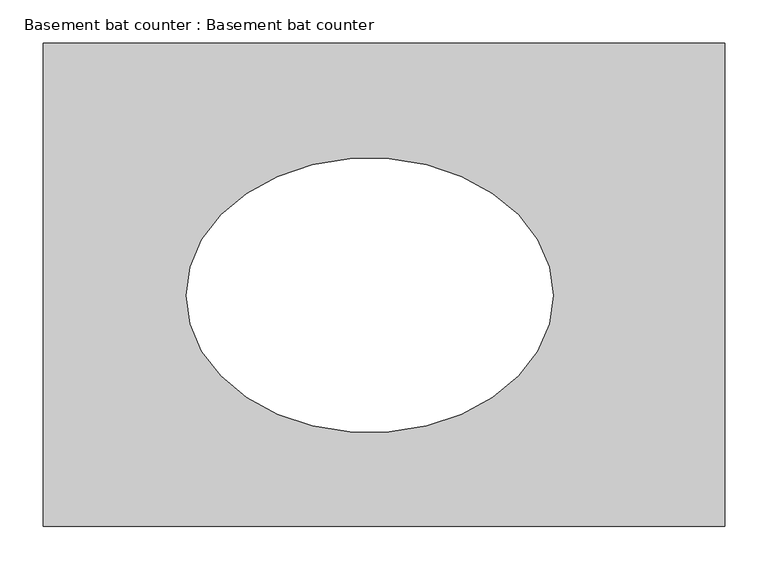
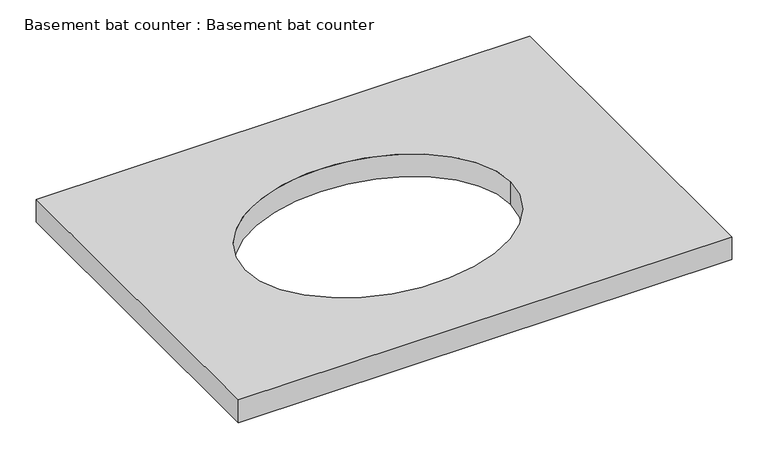
"""IFC4 building model written with IfcOpenShell, lengths in millimetres: furniture geometry, Basement bat counter : Basement bat counter."""

from ifc_helpers import new_model, si_unit, point, frame, origin, place, context, project, spatial, ellipse_curve, trimmed, source, transform, mapped, element, save
from ifc_brep_helpers import plane_surface, extruded_surface, advanced_brep


def basement_bat_counter_basement_bat_counter_ad1241f1(model_context):
    return source(origin(), model_context, "Body", "AdvancedBrep", [
        advanced_brep(
        [(963.0652851, 15145.821245, -2755.9), (963.0652851, 15704.621245, -2755.9), (1750.4652851, 15704.621245, -2755.9), (1750.4652851, 15145.821245, -2755.9), (1552.1234749, 15413.0467639, -2755.9), (1128.1234749, 15413.0467639, -2755.9), (963.0652851, 15145.821245, -2717.8), (1750.4652851, 15145.821245, -2717.8), (1750.4652851, 15704.621245, -2717.8), (963.0652851, 15704.621245, -2717.8), (1552.1234749, 15413.0467639, -2717.8), (1128.1234749, 15413.0467639, -2717.8)],
        [
            (0, 1),
            (1, 2),
            (2, 3),
            (3, 0),
            (4, 5, ellipse_curve(frame((1340.1234749, 15413.0467639, -2755.9), z_axis=(0.0, 0.0, 1.0), x_axis=(-1.0, 0.0, 0.0)), 212.0, 158.7697221)),
            (5, 4, ellipse_curve(frame((1340.1234749, 15413.0467639, -2755.9), z_axis=(0.0, 0.0, 1.0), x_axis=(-1.0, 0.0, 0.0)), 212.0, 158.7697221)),
            (6, 7),
            (7, 8),
            (8, 9),
            (9, 6),
            (10, 11, ellipse_curve(frame((1340.1234749, 15413.0467639, -2717.8), z_axis=(0.0, 0.0, -1.0), x_axis=(-1.0, 0.0, 0.0)), 212.0, 158.7697221)),
            (11, 10, ellipse_curve(frame((1340.1234749, 15413.0467639, -2717.8), z_axis=(0.0, 0.0, -1.0), x_axis=(-1.0, 0.0, 0.0)), 212.0, 158.7697221)),
            (6, 0),
            (3, 7),
            (2, 8),
            (1, 9),
            (10, 4),
            (5, 11),
        ],
        [
            plane_surface(frame((963.0652851, 15145.821245, -2755.9), z_axis=(0.0, 0.0, -1.0), x_axis=(-1.0, 0.0, 0.0))),
            plane_surface(frame((963.0652851, 15145.821245, -2717.8), z_axis=(0.0, 0.0, 1.0), x_axis=(1.0, 0.0, 0.0))),
            plane_surface(frame((963.0652851, 15145.821245, -2717.8), z_axis=(0.0, -1.0, 0.0), x_axis=(0.0, 0.0, -1.0))),
            plane_surface(frame((1750.4652851, 15145.821245, -2717.8), z_axis=(1.0, 0.0, 0.0), x_axis=(0.0, 0.0, -1.0))),
            plane_surface(frame((1750.4652851, 15704.621245, -2717.8), z_axis=(0.0, 1.0, 0.0), x_axis=(0.0, 0.0, -1.0))),
            plane_surface(frame((963.0652851, 15704.621245, -2717.8), z_axis=(-1.0, 0.0, 0.0), x_axis=(0.0, 0.0, -1.0))),
            extruded_surface(trimmed(ellipse_curve(frame((1340.1234749, 15413.0467639, -3594.1), z_axis=(0.0, 0.0, -1.0), x_axis=(-1.0, 0.0, 0.0)), 212.0, 158.7697221), [point((1552.1234749, 15413.0467639, -3594.1))], [point((1128.1234749, 15413.0467639, -3594.1))], True, "CARTESIAN"), (0.0, 0.0, 38.09999999999991), 38.09999999999991),
            extruded_surface(trimmed(ellipse_curve(frame((1340.1234749, 15413.0467639, -3594.1), z_axis=(0.0, 0.0, -1.0), x_axis=(-1.0, 0.0, 0.0)), 212.0, 158.7697221), [point((1128.1234749, 15413.0467639, -3594.1))], [point((1552.1234749, 15413.0467639, -3594.1))], True, "CARTESIAN"), (0.0, 0.0, 38.09999999999991), 38.09999999999991),
        ],
        [
            (0, [[1, 2, 3, 4], [5, 6]]),
            (1, [[7, 8, 9, 10], [11, 12]]),
            (2, [[-7, 13, -4, 14]]),
            (3, [[-8, -14, -3, 15]]),
            (4, [[-9, -15, -2, 16]]),
            (5, [[-10, -16, -1, -13]]),
            (6, [[-11, 17, -6, 18]]),
            (7, [[-12, -18, -5, -17]]),
        ],
    ),
    ])


if __name__ == "__main__":
    model = new_model("IFC4")
    model_context = context("Model", 3, world=origin())
    ifc_project = project(units=[si_unit("LENGTHUNIT", "METRE", prefix="MILLI")], contexts=[model_context])
    site = spatial("IfcSite", under=ifc_project)
    building = spatial("IfcBuilding", under=site)
    placement = place(None, origin())
    basement_bat_counter_basement_bat_counter_shape = basement_bat_counter_basement_bat_counter_ad1241f1(model_context)
    element("IfcFurniture", 1, ObjectType="Basement bat counter : Basement bat counter", at=placement, inside=building, context=model_context, shape_type="MappedRepresentation", body=[
        mapped(basement_bat_counter_basement_bat_counter_shape, transform((0.0, 0.0, 0.0), x_axis=(1.0, 0.0, 0.0), y_axis=(0.0, 1.0, 0.0), z_axis=(0.0, 0.0, 1.0))),
    ])
    save(model, "model.ifc")

# Revit data of these elements
# Type "Basement bat counter : Basement bat counter"
#   COBie.Type = no
# Element 1 (IfcFurniture, "Basement bat counter : Basement bat counter")
#   Materials on its faces: "Corian - Dusk"
# Materials
#   "Corian - Dusk": class "Plastic", colour RGB 75 95 146, transparency 0, Manufacturer = "Corning", Cost = 0
